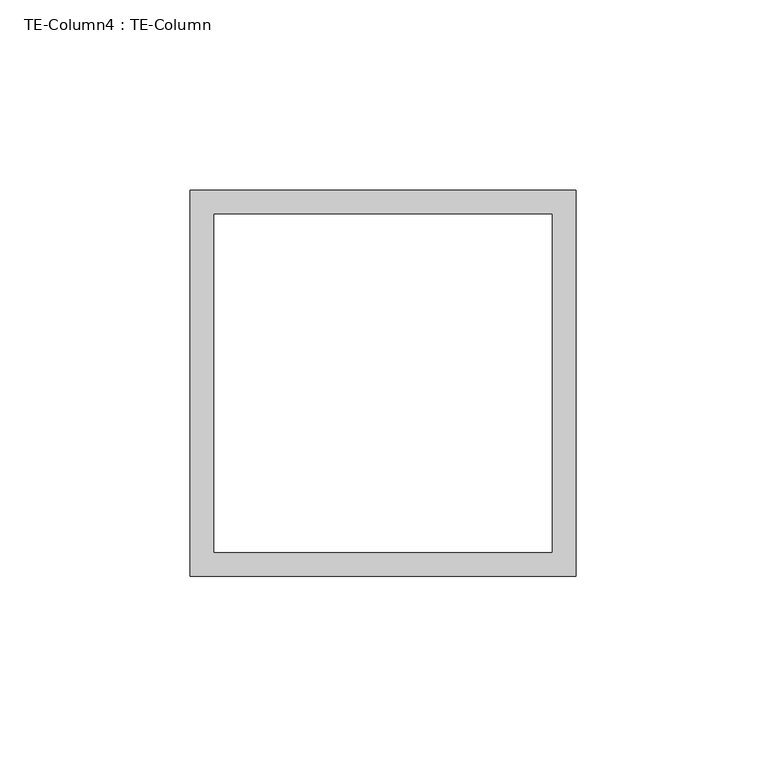
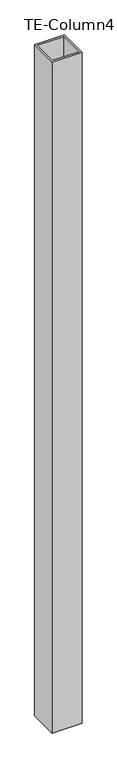
"""IFC4 building model written with IfcOpenShell, lengths in millimetres: proxy geometry, TE-Column4 : TE-Column."""

from ifc_helpers import new_model, si_unit, frame, origin, place, context, project, spatial, polyline, outline, extrude, source, transform, mapped, element, save


def te_column4_te_column_72f26b47(model_context):
    return source(origin(), model_context, "Body", "SweptSolid", [
        extrude(outline(polyline([(590318.6434739, -534093.4913841), (590217.0434739, -534093.4913841), (590217.0434739, -533991.8913841), (590318.6434739, -533991.8913841), (590318.6434739, -534093.4913841)]), holes=[polyline([(590312.2934739, -533998.2413841), (590223.3934739, -533998.2413841), (590223.3934739, -534087.1413841), (590312.2934739, -534087.1413841), (590312.2934739, -533998.2413841)])]), frame((0.0, 0.0, 28.575), z_axis=(0.0, 0.0, 1.0), x_axis=(1.0, 0.0, 0.0)), (0.0, 0.0, 1.0), 2406.65),
    ])


if __name__ == "__main__":
    model = new_model("IFC4")
    model_context = context("Model", 3, world=origin())
    ifc_project = project(units=[si_unit("LENGTHUNIT", "METRE", prefix="MILLI")], contexts=[model_context])
    site = spatial("IfcSite", under=ifc_project)
    building = spatial("IfcBuilding", under=site)
    placement = place(None, origin())
    te_column4_te_column_shape = te_column4_te_column_72f26b47(model_context)
    element("IfcBuildingElementProxy", 1, Name="TE-Column4 : TE-Column", ObjectType="TE-Column4 : TE-Column", at=placement, inside=building, context=model_context, shape_type="MappedRepresentation", body=[
        mapped(te_column4_te_column_shape, transform((0.0, 0.0, 0.0), x_axis=(1.0, 0.0, 0.0), y_axis=(0.0, 1.0, 0.0), z_axis=(0.0, 0.0, 1.0))),
    ])
    save(model, "model.ifc")

# Revit data of these elements
# Element 1 (IfcBuildingElementProxy, "TE-Column4 : TE-Column")
#   Materials on its faces: "4\"X4\" GALV. HSS TUBING"
# Materials
#   "4\"X4\" GALV. HSS TUBING": class "Generic", colour RGB 211 211 207, transparency 0, Cost = 0
